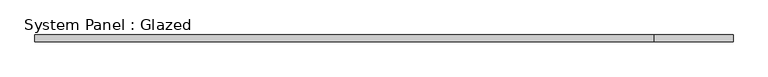
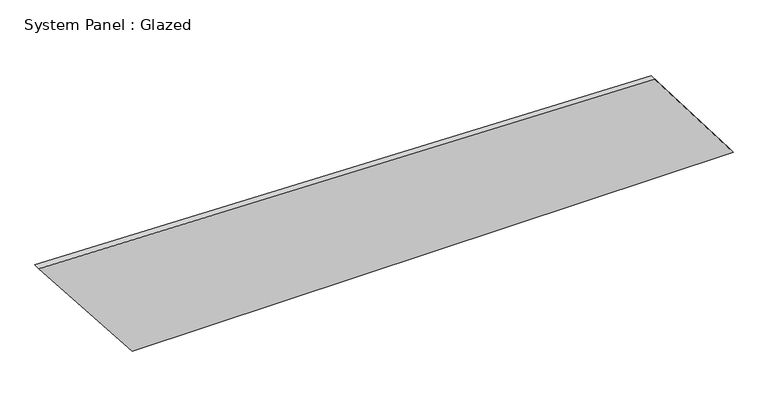
"""IFC4 building model written with IfcOpenShell, lengths in millimetres: plate geometry, System Panel : Glazed."""

from ifc_helpers import new_model, si_unit, frame, origin, place, context, project, spatial, polyline, outline, extrude, source, transform, mapped, element, save


def system_panel_glazed_ffbfcff5(model_context):
    return source(origin(), model_context, "Body", "SweptSolid", [
        extrude(outline(polyline([(0.0, -953.5908288), (0.0, 1304.7464291), (391.8882913, 1010.9060534), (450.6706626, -1304.7464291), (0.0, -953.5908288)])), frame((0.0, -49.5, 0.0), z_axis=(0.0, 1.0, 0.0), x_axis=(0.0, 0.0, 1.0)), (0.0, 0.0, 1.0), 25.0),
    ])


if __name__ == "__main__":
    model = new_model("IFC4")
    model_context = context("Model", 3, world=origin())
    ifc_project = project(units=[si_unit("LENGTHUNIT", "METRE", prefix="MILLI")], contexts=[model_context])
    site = spatial("IfcSite", under=ifc_project)
    building = spatial("IfcBuilding", under=site)
    placement = place(None, origin())
    system_panel_glazed_shape = system_panel_glazed_ffbfcff5(model_context)
    element("IfcPlate", 1, ObjectType="System Panel : Glazed", at=placement, inside=building, context=model_context, shape_type="MappedRepresentation", body=[
        mapped(system_panel_glazed_shape, transform((0.0, 0.0, 0.0), x_axis=(1.0, 0.0, 0.0), y_axis=(0.0, 1.0, 0.0), z_axis=(0.0, 0.0, 1.0))),
    ])
    save(model, "model.ifc")

# Revit data of these elements
# Element 1 (IfcPlate, "System Panel : Glazed")
#   Materials on its faces: "Glass, Clear Glazing"
# Materials
#   "Glass, Clear Glazing": class "Glass", colour RGB 247 249 248, transparency 0.85, Description = "Clear glazing", Cost = 0
